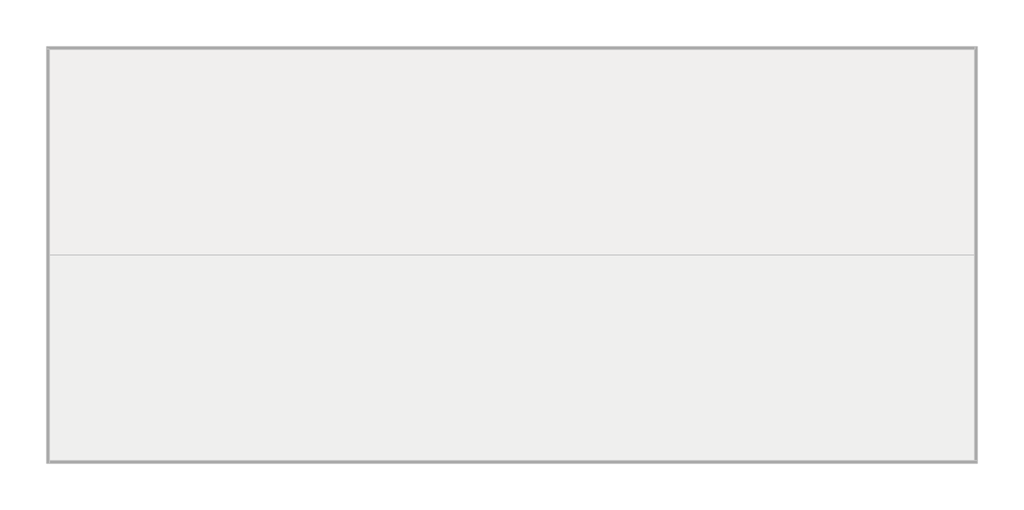
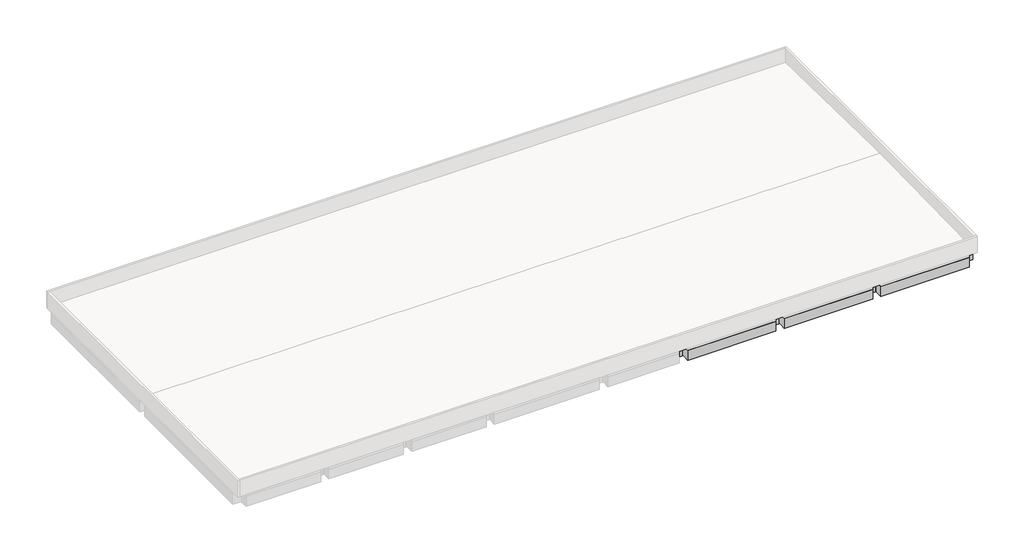
# One storey, part 2 of 2: 37 beams.
"""IFC4 building model written with IfcOpenShell, lengths in millimetres."""

from ifc_helpers import new_model, si_unit, origin, place, context, project, spatial, faceted_brep, element, save

model = new_model("IFC4")

# Units and contexts
model_context = context("Model", 3, world=origin())
ifc_project = project(units=[si_unit("LENGTHUNIT", "METRE", prefix="MILLI")], contexts=[model_context])

# Site, building, storey
site = spatial("IfcSite", under=ifc_project)
building = spatial("IfcBuilding", under=site)
storey = spatial("IfcBuildingStorey", under=building, Name="TOC", Elevation=7649.9618634)

# Beams
placement = place(None, origin())
element("IfcBeam", 1, ObjectType="RC Beam_Rectangular : H_SB_AR_S16_B600xH900_RG9", at=placement, inside=storey, context=model_context, shape_type="Brep", body=[
    faceted_brep([(300.0, 24199.5208589, 6749.9618634), (300.0, 23749.5208589, 6749.9618634), (300.0, 23599.5208589, 6749.9618634), (300.0, 23599.5208589, 7499.9618634), (300.0, 24199.5208589, 7499.9618634), (5700.0, 23599.5208589, 6749.9618634), (5700.0, 23749.5208589, 6749.9618634), (5700.0, 24199.5208589, 6749.9618634), (5700.0, 24199.5208589, 7499.9618634), (5700.0, 23599.5208589, 7499.9618634), (2800.0, 23599.5208589, 7499.9618634), (3200.0, 23599.5208589, 7499.9618634), (2800.0, 23599.5208589, 6749.9618634), (3200.0, 23599.5208589, 6749.9618634)], [[[0, 1, 2, 3, 4]], [[5, 6, 7, 8, 9]], [[4, 3, 10, 11, 9, 8]], [[2, 12, 13, 5, 9, 11, 10, 3]], [[2, 1, 0, 7, 6, 5, 13, 12]], [[7, 0, 4, 8]]]),
])
element("IfcBeam", 2, ObjectType="RC Beam_Rectangular : H_SB_AR_S16_B600xH900_RG9", at=placement, inside=storey, context=model_context, shape_type="Brep", body=[
    faceted_brep([(6300.0, 24199.5208589, 6749.9618634), (6300.0, 23749.5208589, 6749.9618634), (6300.0, 23599.5208589, 6749.9618634), (6300.0, 23599.5208589, 7499.9618634), (6300.0, 24199.5208589, 7499.9618634), (11700.0, 23599.5208589, 6749.9618634), (11700.0, 23749.5208589, 6749.9618634), (11700.0, 24199.5208589, 6749.9618634), (11700.0, 24199.5208589, 7499.9618634), (11700.0, 23599.5208589, 7499.9618634), (8800.0, 23599.5208589, 7499.9618634), (9200.0, 23599.5208589, 7499.9618634), (8800.0, 23599.5208589, 6749.9618634), (9200.0, 23599.5208589, 6749.9618634)], [[[0, 1, 2, 3, 4]], [[5, 6, 7, 8, 9]], [[4, 3, 10, 11, 9, 8]], [[2, 12, 13, 5, 9, 11, 10, 3]], [[2, 1, 0, 7, 6, 5, 13, 12]], [[7, 0, 4, 8]]]),
])
element("IfcBeam", 3, ObjectType="RC Beam_Rectangular : H_SB_AR_S16_B600xH900_RG9", at=placement, inside=storey, context=model_context, shape_type="Brep", body=[
    faceted_brep([(12300.0, 24199.5208589, 6749.9618634), (12300.0, 23749.5208589, 6749.9618634), (12300.0, 23599.5208589, 6749.9618634), (12300.0, 23599.5208589, 7499.9618634), (12300.0, 24199.5208589, 7499.9618634), (17700.0, 23599.5208589, 6749.9618634), (17700.0, 23749.5208589, 6749.9618634), (17700.0, 24199.5208589, 6749.9618634), (17700.0, 24199.5208589, 7499.9618634), (17700.0, 23599.5208589, 7499.9618634), (14800.0, 23599.5208589, 7499.9618634), (15200.0, 23599.5208589, 7499.9618634), (14800.0, 23599.5208589, 6749.9618634), (15200.0, 23599.5208589, 6749.9618634)], [[[0, 1, 2, 3, 4]], [[5, 6, 7, 8, 9]], [[4, 3, 10, 11, 9, 8]], [[2, 12, 13, 5, 9, 11, 10, 3]], [[2, 1, 0, 7, 6, 5, 13, 12]], [[7, 0, 4, 8]]]),
])
element("IfcBeam", 4, ObjectType="RC Beam_Rectangular : H_SB_AR_S16_B600xH900_RG9", at=placement, inside=storey, context=model_context, shape_type="Brep", body=[
    faceted_brep([(18300.0, 24199.5208589, 6749.9618634), (18300.0, 23749.5208589, 6749.9618634), (18300.0, 23599.5208589, 6749.9618634), (18300.0, 23599.5208589, 7499.9618634), (18300.0, 24199.5208589, 7499.9618634), (25900.0, 23599.5208589, 6749.9618634), (25900.0, 23749.5208589, 6749.9618634), (25900.0, 24199.5208589, 6749.9618634), (25900.0, 24199.5208589, 7499.9618634), (25900.0, 23599.5208589, 7499.9618634), (21800.0, 23599.5208589, 7499.9618634), (22400.0, 23599.5208589, 7499.9618634), (21800.0, 23599.5208589, 6749.9618634), (22400.0, 23599.5208589, 6749.9618634)], [[[0, 1, 2, 3, 4]], [[5, 6, 7, 8, 9]], [[4, 3, 10, 11, 9, 8]], [[2, 12, 13, 5, 9, 11, 10, 3]], [[2, 1, 0, 7, 6, 5, 13, 12]], [[7, 0, 4, 8]]]),
])
element("IfcBeam", 5, ObjectType="RC Beam_Rectangular : H_SB_AR_S16_B600xH900_RG9", at=placement, inside=storey, context=model_context, shape_type="Brep", body=[
    faceted_brep([(26500.0, 24199.5208589, 6749.9618634), (26500.0, 23749.5208589, 6749.9618634), (26500.0, 23599.5208589, 6749.9618634), (26500.0, 23599.5208589, 7499.9618634), (26500.0, 24199.5208589, 7499.9618634), (31700.0, 23599.5208589, 6749.9618634), (31700.0, 23749.5208589, 6749.9618634), (31700.0, 24199.5208589, 6749.9618634), (31700.0, 24199.5208589, 7499.9618634), (31700.0, 23599.5208589, 7499.9618634), (28800.0, 23599.5208589, 7499.9618634), (29400.0, 23599.5208589, 7499.9618634), (28800.0, 23599.5208589, 6749.9618634), (29400.0, 23599.5208589, 6749.9618634)], [[[0, 1, 2, 3, 4]], [[5, 6, 7, 8, 9]], [[4, 3, 10, 11, 9, 8]], [[2, 12, 13, 5, 9, 11, 10, 3]], [[2, 1, 0, 7, 6, 5, 13, 12]], [[7, 0, 4, 8]]]),
])
element("IfcBeam", 6, ObjectType="RC Beam_Rectangular : H_SB_AR_S16_B600xH900_RG9", at=placement, inside=storey, context=model_context, shape_type="Brep", body=[
    faceted_brep([(32300.0, 24199.5208589, 6749.9618634), (32300.0, 23749.5208589, 6749.9618634), (32300.0, 23599.5208589, 6749.9618634), (32300.0, 23599.5208589, 7499.9618634), (32300.0, 24199.5208589, 7499.9618634), (38700.0, 23599.5208589, 6749.9618634), (38700.0, 23749.5208589, 6749.9618634), (38700.0, 24199.5208589, 6749.9618634), (38700.0, 24199.5208589, 7499.9618634), (38700.0, 23599.5208589, 7499.9618634), (33250.0, 23599.5208589, 7499.9618634), (33450.0, 23599.5208589, 7499.9618634), (35200.0, 23599.5208589, 7499.9618634), (35800.0, 23599.5208589, 7499.9618634), (35200.0, 23599.5208589, 6749.9618634), (35800.0, 23599.5208589, 6749.9618634)], [[[0, 1, 2, 3, 4]], [[5, 6, 7, 8, 9]], [[4, 3, 10, 11, 12, 13, 9, 8]], [[2, 14, 15, 5, 9, 13, 12, 11, 10, 3]], [[2, 1, 0, 7, 6, 5, 15, 14]], [[7, 0, 4, 8]]]),
])
element("IfcBeam", 7, ObjectType="RC Beam_Rectangular : H_SB_AR_S16_B600xH900_RG9", at=placement, inside=storey, context=model_context, shape_type="Brep", body=[
    faceted_brep([(39300.0, 24199.5208589, 6749.9618634), (39300.0, 23749.5208589, 6749.9618634), (39300.0, 23599.5208589, 6749.9618634), (39300.0, 23599.5208589, 7499.9618634), (39300.0, 24199.5208589, 7499.9618634), (45700.0, 23599.5208589, 6749.9618634), (45700.0, 23749.5208589, 6749.9618634), (45700.0, 24199.5208589, 6749.9618634), (45700.0, 24199.5208589, 7499.9618634), (45700.0, 23599.5208589, 7499.9618634), (42200.0, 23599.5208589, 7499.9618634), (42800.0, 23599.5208589, 7499.9618634), (43500.0, 23599.5208589, 7499.9618634), (43700.0, 23599.5208589, 7499.9618634), (42200.0, 23599.5208589, 6749.9618634), (42800.0, 23599.5208589, 6749.9618634)], [[[0, 1, 2, 3, 4]], [[5, 6, 7, 8, 9]], [[4, 3, 10, 11, 12, 13, 9, 8]], [[2, 14, 15, 5, 9, 13, 12, 11, 10, 3]], [[2, 1, 0, 7, 6, 5, 15, 14]], [[7, 0, 4, 8]]]),
])
element("IfcBeam", 8, ObjectType="RC Beam_Rectangular : H_SB_AR_S16_B600xH900_RG9", at=placement, inside=storey, context=model_context, shape_type="Brep", body=[
    faceted_brep([(46300.0, 24199.5208589, 6749.9618634), (46300.0, 23749.5208589, 6749.9618634), (46300.0, 23599.5208589, 6749.9618634), (46300.0, 23599.5208589, 7499.9618634), (46300.0, 24199.5208589, 7499.9618634), (52700.0, 23599.5208589, 6749.9618634), (52700.0, 23749.5208589, 6749.9618634), (52700.0, 24199.5208589, 6749.9618634), (52700.0, 24199.5208589, 7499.9618634), (52700.0, 23599.5208589, 7499.9618634), (48900.0, 23599.5208589, 7499.9618634), (49100.0, 23599.5208589, 7499.9618634), (49200.0, 23599.5208589, 7499.9618634), (49800.0, 23599.5208589, 7499.9618634), (52574.0, 23599.5208589, 7499.9618634), (49200.0, 23599.5208589, 6749.9618634), (49800.0, 23599.5208589, 6749.9618634)], [[[0, 1, 2, 3, 4]], [[5, 6, 7, 8, 9]], [[4, 3, 10, 11, 12, 13, 14, 9, 8]], [[2, 15, 16, 5, 9, 14, 13, 12, 11, 10, 3]], [[2, 1, 0, 7, 6, 5, 16, 15]], [[7, 0, 4, 8]]]),
])
element("IfcBeam", 9, ObjectType="RC Beam_Rectangular : H_SB_AR_S16_B600xH900_RG5", at=placement, inside=storey, context=model_context, shape_type="Brep", body=[
    faceted_brep([(32300.0, 8599.5208589, 6749.9618634), (32300.0, 8399.5208589, 6749.9618634), (32300.0, 7999.5208589, 6749.9618634), (32300.0, 7999.5208589, 7499.9618634), (32300.0, 8599.5208589, 7499.9618634), (38700.0, 7999.5208589, 6749.9618634), (38700.0, 8599.5208589, 6749.9618634), (38700.0, 8599.5208589, 7499.9618634), (38700.0, 7999.5208589, 7499.9618634), (35200.0, 7999.5208589, 7499.9618634), (35800.0, 7999.5208589, 7499.9618634), (36500.0, 7999.5208589, 7499.9618634), (36700.0, 7999.5208589, 7499.9618634), (36700.0, 8599.5208589, 7499.9618634), (36500.0, 8599.5208589, 7499.9618634), (35800.0, 8599.5208589, 7499.9618634), (35200.0, 8599.5208589, 7499.9618634), (33450.0, 8599.5208589, 7499.9618634), (33250.0, 8599.5208589, 7499.9618634), (35200.0, 7999.5208589, 6749.9618634), (35800.0, 7999.5208589, 6749.9618634), (36500.0, 7999.5208589, 6749.9618634), (36700.0, 7999.5208589, 6749.9618634), (35200.0, 8599.5208589, 6749.9618634), (35800.0, 8599.5208589, 6749.9618634), (36500.0, 8599.5208589, 6749.9618634), (36700.0, 8599.5208589, 6749.9618634)], [[[0, 1, 2, 3, 4]], [[5, 6, 7, 8]], [[4, 3, 9, 10, 11, 12, 8, 7, 13, 14, 15, 16, 17, 18]], [[2, 19, 20, 21, 22, 5, 8, 12, 11, 10, 9, 3]], [[2, 1, 0, 23, 24, 25, 26, 6, 5, 22, 21, 20, 19]], [[6, 26, 25, 24, 23, 0, 4, 18, 17, 16, 15, 14, 13, 7]]]),
])
element("IfcBeam", 10, ObjectType="RC Beam_Rectangular : H_SB_AR_S16_B600xH900_RG5", at=placement, inside=storey, context=model_context, shape_type="Brep", body=[
    faceted_brep([(39300.0, 8599.5208589, 6749.9618634), (39300.0, 8404.5208589, 6749.9618634), (39300.0, 8204.5208589, 6749.9618634), (39300.0, 7999.5208589, 6749.9618634), (39300.0, 7999.5208589, 7499.9618634), (39300.0, 8599.5208589, 7499.9618634), (45700.0, 7999.5208589, 6749.9618634), (45700.0, 8399.5208589, 6749.9618634), (45700.0, 8599.5208589, 6749.9618634), (45700.0, 8599.5208589, 7499.9618634), (45700.0, 7999.5208589, 7499.9618634), (41925.0, 7999.5208589, 7499.9618634), (42125.0, 7999.5208589, 7499.9618634), (42200.0, 7999.5208589, 7499.9618634), (42800.0, 7999.5208589, 7499.9618634), (43200.0, 7999.5208589, 7499.9618634), (43400.0, 7999.5208589, 7499.9618634), (45440.0, 7999.5208589, 7499.9618634), (45640.0, 7999.5208589, 7499.9618634), (42800.0, 8599.5208589, 7499.9618634), (42200.0, 8599.5208589, 7499.9618634), (41925.0, 7999.5208589, 6749.9618634), (42125.0, 7999.5208589, 6749.9618634), (42200.0, 7999.5208589, 6749.9618634), (42800.0, 7999.5208589, 6749.9618634), (43200.0, 7999.5208589, 6749.9618634), (43400.0, 7999.5208589, 6749.9618634), (45440.0, 7999.5208589, 6749.9618634), (45640.0, 7999.5208589, 6749.9618634), (42200.0, 8599.5208589, 6749.9618634), (42800.0, 8599.5208589, 6749.9618634), (45440.0, 8599.5208589, 6749.9618634), (45640.0, 8599.5208589, 6749.9618634)], [[[0, 1, 2, 3, 4, 5]], [[6, 7, 8, 9, 10]], [[5, 4, 11, 12, 13, 14, 15, 16, 17, 18, 10, 9, 19, 20]], [[3, 21, 22, 23, 24, 25, 26, 27, 28, 6, 10, 18, 17, 16, 15, 14, 13, 12, 11, 4]], [[3, 2, 1, 0, 29, 30, 31, 32, 8, 7, 6, 28, 27, 26, 25, 24, 23, 22, 21]], [[8, 32, 31, 30, 29, 0, 5, 20, 19, 9]]]),
])
element("IfcBeam", 11, ObjectType="RC Beam_Rectangular : H_SB_AR_S16_B600xH900_RG5", at=placement, inside=storey, context=model_context, shape_type="Brep", body=[
    faceted_brep([(46300.0, 8599.5208589, 6749.9618634), (46300.0, 8399.5208589, 6749.9618634), (46300.0, 7999.5208589, 6749.9618634), (46300.0, 7999.5208589, 7499.9618634), (46300.0, 8599.5208589, 7499.9618634), (52700.0, 7999.5208589, 6749.9618634), (52700.0, 8399.5208589, 6749.9618634), (52700.0, 8599.5208589, 6749.9618634), (52700.0, 8599.5208589, 7499.9618634), (52700.0, 7999.5208589, 7499.9618634), (49200.0, 7999.5208589, 7499.9618634), (49800.0, 7999.5208589, 7499.9618634), (52574.0, 7999.5208589, 7499.9618634), (52574.0, 8599.5208589, 7499.9618634), (50725.0, 8599.5208589, 7499.9618634), (50525.0, 8599.5208589, 7499.9618634), (49800.0, 8599.5208589, 7499.9618634), (49200.0, 8599.5208589, 7499.9618634), (49200.0, 7999.5208589, 6749.9618634), (49800.0, 7999.5208589, 6749.9618634), (52574.0, 7999.5208589, 6749.9618634), (49200.0, 8599.5208589, 6749.9618634), (49800.0, 8599.5208589, 6749.9618634)], [[[0, 1, 2, 3, 4]], [[5, 6, 7, 8, 9]], [[4, 3, 10, 11, 12, 9, 8, 13, 14, 15, 16, 17]], [[2, 18, 19, 20, 5, 9, 12, 11, 10, 3]], [[2, 1, 0, 21, 22, 7, 6, 5, 20, 19, 18]], [[7, 22, 21, 0, 4, 17, 16, 15, 14, 13, 8]]]),
])
element("IfcBeam", 12, ObjectType="RC Beam_Rectangular : H_SB_AR_S16_B600xH900_RG9", at=placement, inside=storey, context=model_context, shape_type="Brep", body=[
    faceted_brep([(32300.0, 799.5208589, 6749.9618634), (32300.0, 649.5208589, 6749.9618634), (32300.0, 199.5208589, 6749.9618634), (32300.0, 199.5208589, 7499.9618634), (32300.0, 799.5208589, 7499.9618634), (38700.0, 199.5208589, 6749.9618634), (38700.0, 649.5208589, 6749.9618634), (38700.0, 799.5208589, 6749.9618634), (38700.0, 799.5208589, 7499.9618634), (38700.0, 199.5208589, 7499.9618634), (36700.0, 799.5208589, 7499.9618634), (36500.0, 799.5208589, 7499.9618634), (35800.0, 799.5208589, 7499.9618634), (35200.0, 799.5208589, 7499.9618634), (35200.0, 799.5208589, 6749.9618634), (35800.0, 799.5208589, 6749.9618634)], [[[0, 1, 2, 3, 4]], [[5, 6, 7, 8, 9]], [[4, 3, 9, 8, 10, 11, 12, 13]], [[2, 5, 9, 3]], [[2, 1, 0, 14, 15, 7, 6, 5]], [[7, 15, 14, 0, 4, 13, 12, 11, 10, 8]]]),
])
element("IfcBeam", 13, ObjectType="RC Beam_Rectangular : H_SB_AR_S16_B600xH900_RG9", at=placement, inside=storey, context=model_context, shape_type="Brep", body=[
    faceted_brep([(39300.0, 799.5208589, 6749.9618634), (39300.0, 649.5208589, 6749.9618634), (39300.0, 199.5208589, 6749.9618634), (39300.0, 199.5208589, 7499.9618634), (39300.0, 799.5208589, 7499.9618634), (45700.0, 199.5208589, 6749.9618634), (45700.0, 649.5208589, 6749.9618634), (45700.0, 799.5208589, 6749.9618634), (45700.0, 799.5208589, 7499.9618634), (45700.0, 199.5208589, 7499.9618634), (43400.0, 799.5208589, 7499.9618634), (43200.0, 799.5208589, 7499.9618634), (42800.0, 799.5208589, 7499.9618634), (42200.0, 799.5208589, 7499.9618634), (42200.0, 799.5208589, 6749.9618634), (42800.0, 799.5208589, 6749.9618634)], [[[0, 1, 2, 3, 4]], [[5, 6, 7, 8, 9]], [[4, 3, 9, 8, 10, 11, 12, 13]], [[2, 5, 9, 3]], [[2, 1, 0, 14, 15, 7, 6, 5]], [[7, 15, 14, 0, 4, 13, 12, 11, 10, 8]]]),
])
element("IfcBeam", 14, ObjectType="RC Beam_Rectangular : H_SB_AR_S16_B600xH900_RG9", at=placement, inside=storey, context=model_context, shape_type="Brep", body=[
    faceted_brep([(46300.0, 799.5208589, 6749.9618634), (46300.0, 649.5208589, 6749.9618634), (46300.0, 199.5208589, 6749.9618634), (46300.0, 199.5208589, 7499.9618634), (46300.0, 799.5208589, 7499.9618634), (52700.0, 199.5208589, 6749.9618634), (52700.0, 649.5208589, 6749.9618634), (52700.0, 799.5208589, 6749.9618634), (52700.0, 799.5208589, 7499.9618634), (52700.0, 199.5208589, 7499.9618634), (49800.0, 799.5208589, 7499.9618634), (49200.0, 799.5208589, 7499.9618634), (46800.0, 799.5208589, 7499.9618634), (46600.0, 799.5208589, 7499.9618634), (49200.0, 799.5208589, 6749.9618634), (49800.0, 799.5208589, 6749.9618634)], [[[0, 1, 2, 3, 4]], [[5, 6, 7, 8, 9]], [[4, 3, 9, 8, 10, 11, 12, 13]], [[2, 5, 9, 3]], [[2, 1, 0, 14, 15, 7, 6, 5]], [[7, 15, 14, 0, 4, 13, 12, 11, 10, 8]]]),
])
element("IfcBeam", 15, ObjectType="RC Beam_Rectangular : H_SB_AR_S16_B400xH900_RG1", at=placement, inside=storey, context=model_context, shape_type="Brep", body=[
    faceted_brep([(6200.0, 23599.5208589, 7499.9618634), (5800.0, 23599.5208589, 7499.9618634), (5800.0, 23473.5208589, 7499.9618634), (5800.0, 12499.5208589, 7499.9618634), (6200.0, 12499.5208589, 7499.9618634), (6200.0, 23473.5208589, 7499.9618634), (6200.0, 23599.5208589, 6749.9618634), (5800.0, 23599.5208589, 6749.9618634), (5800.0, 12499.5208589, 6749.9618634), (6200.0, 12499.5208589, 6749.9618634), (6200.0, 23473.5208589, 6749.9618634), (5800.0, 23473.5208589, 6749.9618634)], [[[0, 1, 2, 3, 4, 5]], [[6, 7, 1, 0]], [[8, 9, 4, 3]], [[9, 10, 6, 0, 5, 4]], [[8, 11, 7, 6, 10, 9]], [[7, 11, 8, 3, 2, 1]]]),
])
element("IfcBeam", 16, ObjectType="RC Beam_Rectangular : H_SB_AR_S16_B400xH900_RG1", at=placement, inside=storey, context=model_context, shape_type="Brep", body=[
    faceted_brep([(12200.0, 23599.5208589, 7499.9618634), (11800.0, 23599.5208589, 7499.9618634), (11800.0, 23473.5208589, 7499.9618634), (11800.0, 12499.5208589, 7499.9618634), (12200.0, 12499.5208589, 7499.9618634), (12200.0, 23473.5208589, 7499.9618634), (12200.0, 23599.5208589, 6749.9618634), (11800.0, 23599.5208589, 6749.9618634), (11800.0, 12499.5208589, 6749.9618634), (12200.0, 12499.5208589, 6749.9618634), (12200.0, 23473.5208589, 6749.9618634), (11800.0, 23473.5208589, 6749.9618634)], [[[0, 1, 2, 3, 4, 5]], [[6, 7, 1, 0]], [[8, 9, 4, 3]], [[9, 10, 6, 0, 5, 4]], [[9, 8, 11, 7, 6, 10]], [[7, 11, 8, 3, 2, 1]]]),
])
element("IfcBeam", 17, ObjectType="RC Beam_Rectangular : H_SB_AR_S16_B600xH900_RG1A", at=placement, inside=storey, context=model_context, shape_type="Brep", body=[
    faceted_brep([(17700.0, 12499.5208589, 6749.9618634), (18100.0, 12499.5208589, 6749.9618634), (18300.0, 12499.5208589, 6749.9618634), (18300.0, 12499.5208589, 7499.9618634), (17700.0, 12499.5208589, 7499.9618634), (18300.0, 23473.5208589, 7499.9618634), (18300.0, 23599.5208589, 7499.9618634), (17700.0, 23599.5208589, 7499.9618634), (17700.0, 23473.5208589, 7499.9618634), (18300.0, 23599.5208589, 6749.9618634), (18100.0, 23599.5208589, 6749.9618634), (17700.0, 23599.5208589, 6749.9618634), (17700.0, 23473.5208589, 6749.9618634)], [[[0, 1, 2, 3, 4]], [[4, 3, 5, 6, 7, 8]], [[9, 10, 11, 7, 6]], [[2, 9, 6, 5, 3]], [[0, 12, 11, 10, 9, 2, 1]], [[11, 12, 0, 4, 8, 7]]]),
])
element("IfcBeam", 18, ObjectType="RC Beam_Rectangular : H_SB_AR_S16_B500xH900_RG2", at=placement, inside=storey, context=model_context, shape_type="Brep", body=[
    faceted_brep([(26450.0, 23599.5208589, 7499.9618634), (25950.0, 23599.5208589, 7499.9618634), (25950.0, 23473.5208589, 7499.9618634), (25950.0, 8599.5208589, 7499.9618634), (26450.0, 8599.5208589, 7499.9618634), (26450.0, 23473.5208589, 7499.9618634), (26450.0, 23599.5208589, 6749.9618634), (25950.0, 23599.5208589, 6749.9618634), (25950.0, 8599.5208589, 6749.9618634), (26450.0, 8599.5208589, 6749.9618634), (26450.0, 23473.5208589, 6749.9618634), (25950.0, 23473.5208589, 6749.9618634)], [[[0, 1, 2, 3, 4, 5]], [[6, 7, 1, 0]], [[8, 9, 4, 3]], [[9, 10, 6, 0, 5, 4]], [[6, 10, 9, 8, 11, 7]], [[7, 11, 8, 3, 2, 1]]]),
])
element("IfcBeam", 19, ObjectType="RC Beam_Rectangular : H_SB_AR_S16_B500xH900_RG3", at=placement, inside=storey, context=model_context, shape_type="Brep", body=[
    faceted_brep([(31750.0, 799.5208589, 7499.9618634), (32250.0, 799.5208589, 7499.9618634), (32250.0, 925.5208589, 7499.9618634), (32250.0, 7999.5208589, 7499.9618634), (31750.0, 7999.5208589, 7499.9618634), (31750.0, 799.5208589, 6749.9618634), (31900.0, 799.5208589, 6749.9618634), (32250.0, 799.5208589, 6749.9618634), (32250.0, 7999.5208589, 6749.9618634), (31900.0, 7999.5208589, 6749.9618634), (31750.0, 7999.5208589, 6749.9618634), (32250.0, 925.5208589, 6749.9618634)], [[[0, 1, 2, 3, 4]], [[5, 6, 7, 1, 0]], [[8, 9, 10, 4, 3]], [[7, 11, 8, 3, 2, 1]], [[5, 10, 9, 8, 11, 7, 6]], [[10, 5, 0, 4]]]),
])
element("IfcBeam", 20, ObjectType="RC Beam_Rectangular : H_SB_AR_S16_B500xH900_RG2", at=placement, inside=storey, context=model_context, shape_type="Brep", body=[
    faceted_brep([(32250.0, 23599.5208589, 7499.9618634), (31750.0, 23599.5208589, 7499.9618634), (31750.0, 23473.5208589, 7499.9618634), (31750.0, 8599.5208589, 7499.9618634), (32250.0, 8599.5208589, 7499.9618634), (32250.0, 23473.5208589, 7499.9618634), (32250.0, 23599.5208589, 6749.9618634), (31750.0, 23599.5208589, 6749.9618634), (31750.0, 8599.5208589, 6749.9618634), (32250.0, 8599.5208589, 6749.9618634), (32250.0, 23473.5208589, 6749.9618634), (31750.0, 23473.5208589, 6749.9618634)], [[[0, 1, 2, 3, 4, 5]], [[6, 7, 1, 0]], [[8, 9, 4, 3]], [[9, 10, 6, 0, 5, 4]], [[8, 11, 7, 6, 10, 9]], [[7, 11, 8, 3, 2, 1]]]),
])
element("IfcBeam", 21, ObjectType="RC Beam_Rectangular : H_SB_AR_S16_B500xH900_RG3", at=placement, inside=storey, context=model_context, shape_type="Brep", body=[
    faceted_brep([(38750.0, 799.5208589, 7499.9618634), (39250.0, 799.5208589, 7499.9618634), (39250.0, 925.5208589, 7499.9618634), (39250.0, 4649.5208589, 7499.9618634), (39250.0, 4849.5208589, 7499.9618634), (39250.0, 7999.5208589, 7499.9618634), (38750.0, 7999.5208589, 7499.9618634), (38750.0, 3543.8249516, 7499.9618634), (38750.0, 3343.8249516, 7499.9618634), (38750.0, 925.5208589, 7499.9618634), (38750.0, 799.5208589, 6749.9618634), (38900.0, 799.5208589, 6749.9618634), (39100.0, 799.5208589, 6749.9618634), (39250.0, 799.5208589, 6749.9618634), (39250.0, 7999.5208589, 6749.9618634), (39100.0, 7999.5208589, 6749.9618634), (38900.0, 7999.5208589, 6749.9618634), (38750.0, 7999.5208589, 6749.9618634), (39250.0, 925.5208589, 6749.9618634), (39250.0, 4649.5208589, 6749.9618634), (39250.0, 4849.5208589, 6749.9618634), (38750.0, 925.5208589, 6749.9618634), (38750.0, 3343.8249516, 6749.9618634), (38750.0, 3543.8249516, 6749.9618634)], [[[0, 1, 2, 3, 4, 5, 6, 7, 8, 9]], [[10, 11, 12, 13, 1, 0]], [[14, 15, 16, 17, 6, 5]], [[13, 18, 19, 20, 14, 5, 4, 3, 2, 1]], [[10, 21, 22, 23, 17, 16, 15, 14, 20, 19, 18, 13, 12, 11]], [[17, 23, 22, 21, 10, 0, 9, 8, 7, 6]]]),
])
element("IfcBeam", 22, ObjectType="RC Beam_Rectangular : H_SB_AR_S16_B500xH900_RG2", at=placement, inside=storey, context=model_context, shape_type="Brep", body=[
    faceted_brep([(39250.0, 23599.5208589, 7499.9618634), (38750.0, 23599.5208589, 7499.9618634), (38750.0, 23473.5208589, 7499.9618634), (38750.0, 11149.5208589, 7499.9618634), (38750.0, 10949.5208589, 7499.9618634), (38750.0, 8599.5208589, 7499.9618634), (39250.0, 8599.5208589, 7499.9618634), (39250.0, 10949.5208589, 7499.9618634), (39250.0, 11149.5208589, 7499.9618634), (39250.0, 23473.5208589, 7499.9618634), (39250.0, 23599.5208589, 6749.9618634), (38750.0, 23599.5208589, 6749.9618634), (38750.0, 8599.5208589, 6749.9618634), (39250.0, 8599.5208589, 6749.9618634), (39250.0, 10949.5208589, 6749.9618634), (39250.0, 11149.5208589, 6749.9618634), (39250.0, 23473.5208589, 6749.9618634), (38750.0, 10949.5208589, 6749.9618634), (38750.0, 11149.5208589, 6749.9618634), (38750.0, 23473.5208589, 6749.9618634)], [[[0, 1, 2, 3, 4, 5, 6, 7, 8, 9]], [[10, 11, 1, 0]], [[12, 13, 6, 5]], [[13, 14, 15, 16, 10, 0, 9, 8, 7, 6]], [[12, 17, 18, 19, 11, 10, 16, 15, 14, 13]], [[11, 19, 18, 17, 12, 5, 4, 3, 2, 1]]]),
])
element("IfcBeam", 23, ObjectType="RC Beam_Rectangular : H_SB_AR_S16_B500xH900_RG3", at=placement, inside=storey, context=model_context, shape_type="Brep", body=[
    faceted_brep([(45750.0, 799.5208589, 7499.9618634), (46250.0, 799.5208589, 7499.9618634), (46250.0, 925.5208589, 7499.9618634), (46250.0, 4649.5208589, 7499.9618634), (46250.0, 4849.5208589, 7499.9618634), (46250.0, 6599.5208589, 7499.9618634), (46250.0, 6799.5208589, 7499.9618634), (46250.0, 7999.5208589, 7499.9618634), (45750.0, 7999.5208589, 7499.9618634), (45750.0, 6799.5208589, 7499.9618634), (45750.0, 6599.5208589, 7499.9618634), (45750.0, 4849.5208589, 7499.9618634), (45750.0, 4649.5208589, 7499.9618634), (45750.0, 925.5208589, 7499.9618634), (45750.0, 799.5208589, 6749.9618634), (46250.0, 799.5208589, 6749.9618634), (46250.0, 7999.5208589, 6749.9618634), (45750.0, 7999.5208589, 6749.9618634), (46250.0, 925.5208589, 6749.9618634), (46250.0, 4649.5208589, 6749.9618634), (46250.0, 4849.5208589, 6749.9618634), (46250.0, 6599.5208589, 6749.9618634), (46250.0, 6799.5208589, 6749.9618634), (45750.0, 925.5208589, 6749.9618634), (45750.0, 4649.5208589, 6749.9618634), (45750.0, 4849.5208589, 6749.9618634), (45750.0, 6599.5208589, 6749.9618634), (45750.0, 6799.5208589, 6749.9618634)], [[[0, 1, 2, 3, 4, 5, 6, 7, 8, 9, 10, 11, 12, 13]], [[14, 15, 1, 0]], [[16, 17, 8, 7]], [[15, 18, 19, 20, 21, 22, 16, 7, 6, 5, 4, 3, 2, 1]], [[14, 23, 24, 25, 26, 27, 17, 16, 22, 21, 20, 19, 18, 15]], [[17, 27, 26, 25, 24, 23, 14, 0, 13, 12, 11, 10, 9, 8]]]),
])
element("IfcBeam", 24, ObjectType="RC Beam_Rectangular : H_SB_AR_S16_B500xH900_RG2", at=placement, inside=storey, context=model_context, shape_type="Brep", body=[
    faceted_brep([(46250.0, 23599.5208589, 7499.9618634), (45750.0, 23599.5208589, 7499.9618634), (45750.0, 19999.5208589, 7499.9618634), (45750.0, 19799.5208589, 7499.9618634), (45750.0, 11149.5208589, 7499.9618634), (45750.0, 10949.5208589, 7499.9618634), (45750.0, 8599.5208589, 7499.9618634), (46250.0, 8599.5208589, 7499.9618634), (46250.0, 10149.5208589, 7499.9618634), (46250.0, 10349.5208589, 7499.9618634), (46250.0, 13899.5208589, 7499.9618634), (46250.0, 14099.5208589, 7499.9618634), (46250.0, 15214.5208589, 7499.9618634), (46250.0, 15414.5208589, 7499.9618634), (46250.0, 16549.5208589, 7499.9618634), (46250.0, 16749.5208589, 7499.9618634), (46250.0, 18399.5208589, 7499.9618634), (46250.0, 18599.5208589, 7499.9618634), (46250.0, 19799.5208589, 7499.9618634), (46250.0, 19999.5208589, 7499.9618634), (46250.0, 23473.5208589, 7499.9618634), (46250.0, 23599.5208589, 6749.9618634), (45900.0, 23599.5208589, 6749.9618634), (45750.0, 23599.5208589, 6749.9618634), (45750.0, 8599.5208589, 6749.9618634), (46250.0, 8599.5208589, 6749.9618634), (46250.0, 10149.5208589, 6749.9618634), (46250.0, 10349.5208589, 6749.9618634), (46250.0, 13899.5208589, 6749.9618634), (46250.0, 14099.5208589, 6749.9618634), (46250.0, 15214.5208589, 6749.9618634), (46250.0, 15414.5208589, 6749.9618634), (46250.0, 16549.5208589, 6749.9618634), (46250.0, 16749.5208589, 6749.9618634), (46250.0, 18399.5208589, 6749.9618634), (46250.0, 18599.5208589, 6749.9618634), (46250.0, 19799.5208589, 6749.9618634), (46250.0, 19999.5208589, 6749.9618634), (46250.0, 23473.5208589, 6749.9618634), (45750.0, 10949.5208589, 6749.9618634), (45750.0, 11149.5208589, 6749.9618634), (45750.0, 19799.5208589, 6749.9618634), (45750.0, 19999.5208589, 6749.9618634)], [[[0, 1, 2, 3, 4, 5, 6, 7, 8, 9, 10, 11, 12, 13, 14, 15, 16, 17, 18, 19, 20]], [[21, 22, 23, 1, 0]], [[24, 25, 7, 6]], [[25, 26, 27, 28, 29, 30, 31, 32, 33, 34, 35, 36, 37, 38, 21, 0, 20, 19, 18, 17, 16, 15, 14, 13, 12, 11, 10, 9, 8, 7]], [[24, 39, 40, 41, 42, 23, 22, 21, 38, 37, 36, 35, 34, 33, 32, 31, 30, 29, 28, 27, 26, 25]], [[23, 42, 41, 40, 39, 24, 6, 5, 4, 3, 2, 1]]]),
])
element("IfcBeam", 25, ObjectType="RC Beam_Rectangular : H_SB_AR_S16_B600xH900_RG8", at=placement, inside=storey, context=model_context, shape_type="Brep", body=[
    faceted_brep([(53300.0, 7999.5208589, 6749.9618634), (52850.0, 7999.5208589, 6749.9618634), (52700.0, 7999.5208589, 6749.9618634), (52700.0, 7999.5208589, 7499.9618634), (53300.0, 7999.5208589, 7499.9618634), (52700.0, 799.5208589, 6749.9618634), (52850.0, 799.5208589, 6749.9618634), (53300.0, 799.5208589, 6749.9618634), (53300.0, 799.5208589, 7499.9618634), (52700.0, 799.5208589, 7499.9618634), (52700.0, 925.5208589, 7499.9618634)], [[[0, 1, 2, 3, 4]], [[5, 6, 7, 8, 9]], [[4, 3, 10, 9, 8]], [[7, 0, 4, 8]], [[2, 1, 0, 7, 6, 5]], [[2, 5, 9, 10, 3]]]),
])
element("IfcBeam", 26, ObjectType="RC Beam_Rectangular : H_SB_AR_S16_B600xH900_RG7", at=placement, inside=storey, context=model_context, shape_type="Brep", body=[
    faceted_brep([(53300.0, 23599.5208589, 6749.9618634), (52850.0, 23599.5208589, 6749.9618634), (52700.0, 23599.5208589, 6749.9618634), (52700.0, 23599.5208589, 7499.9618634), (53300.0, 23599.5208589, 7499.9618634), (52700.0, 8599.5208589, 6749.9618634), (52850.0, 8599.5208589, 6749.9618634), (53300.0, 8599.5208589, 6749.9618634), (53300.0, 8599.5208589, 7499.9618634), (52700.0, 8599.5208589, 7499.9618634), (52700.0, 18599.5208589, 7499.9618634), (52700.0, 18399.5208589, 7499.9618634), (52700.0, 14099.5208589, 7499.9618634), (52700.0, 13899.5208589, 7499.9618634), (52700.0, 11774.5208589, 7499.9618634), (52700.0, 11574.5208589, 7499.9618634)], [[[0, 1, 2, 3, 4]], [[5, 6, 7, 8, 9]], [[4, 3, 10, 11, 12, 13, 14, 15, 9, 8]], [[7, 0, 4, 8]], [[2, 1, 0, 7, 6, 5]], [[2, 5, 9, 15, 14, 13, 12, 11, 10, 3]]]),
])
element("IfcBeam", 27, ObjectType="RC Beam_Rectangular : H_SB_AR_S16_B400xH900_RB1", at=placement, inside=storey, context=model_context, shape_type="Brep", body=[
    faceted_brep([(2800.0, 23599.5208589, 6749.9618634), (2800.0, 23473.5208589, 6749.9618634), (2800.0, 12499.5208589, 6749.9618634), (2800.0, 12499.5208589, 7499.9618634), (2800.0, 23473.5208589, 7499.9618634), (2800.0, 23599.5208589, 7499.9618634), (3200.0, 12499.5208589, 6749.9618634), (3200.0, 23599.5208589, 6749.9618634), (3200.0, 23473.5208589, 6749.9618634), (3200.0, 23599.5208589, 7499.9618634), (3200.0, 23473.5208589, 7499.9618634), (3200.0, 12499.5208589, 7499.9618634)], [[[0, 1, 2, 3, 4, 5]], [[6, 2, 1, 0, 7, 8]], [[6, 8, 7, 9, 10, 11]], [[2, 6, 11, 3]], [[7, 0, 5, 9]], [[5, 4, 3, 11, 10, 9]]]),
])
element("IfcBeam", 28, ObjectType="RC Beam_Rectangular : H_SB_AR_S16_B400xH900_RB1", at=placement, inside=storey, context=model_context, shape_type="Brep", body=[
    faceted_brep([(8800.0, 23599.5208589, 6749.9618634), (8800.0, 23473.5208589, 6749.9618634), (8800.0, 12499.5208589, 6749.9618634), (8800.0, 12499.5208589, 7499.9618634), (8800.0, 23473.5208589, 7499.9618634), (8800.0, 23599.5208589, 7499.9618634), (9200.0, 12499.5208589, 6749.9618634), (9200.0, 23599.5208589, 6749.9618634), (9200.0, 23473.5208589, 6749.9618634), (9200.0, 23599.5208589, 7499.9618634), (9200.0, 23473.5208589, 7499.9618634), (9200.0, 12499.5208589, 7499.9618634)], [[[0, 1, 2, 3, 4, 5]], [[6, 2, 1, 0, 7, 8]], [[6, 8, 7, 9, 10, 11]], [[2, 6, 11, 3]], [[7, 0, 5, 9]], [[5, 4, 3, 11, 10, 9]]]),
])
element("IfcBeam", 29, ObjectType="RC Beam_Rectangular : H_SB_AR_S16_B400xH900_RB1", at=placement, inside=storey, context=model_context, shape_type="Brep", body=[
    faceted_brep([(14800.0, 23599.5208589, 6749.9618634), (14800.0, 23473.5208589, 6749.9618634), (14800.0, 12499.5208589, 6749.9618634), (14800.0, 12499.5208589, 7499.9618634), (14800.0, 23473.5208589, 7499.9618634), (14800.0, 23599.5208589, 7499.9618634), (15200.0, 12499.5208589, 6749.9618634), (15200.0, 23599.5208589, 6749.9618634), (15200.0, 23473.5208589, 6749.9618634), (15200.0, 23599.5208589, 7499.9618634), (15200.0, 23473.5208589, 7499.9618634), (15200.0, 12499.5208589, 7499.9618634)], [[[0, 1, 2, 3, 4, 5]], [[6, 2, 1, 0, 7, 8]], [[6, 8, 7, 9, 10, 11]], [[2, 6, 11, 3]], [[7, 0, 5, 9]], [[5, 4, 3, 11, 10, 9]]]),
])
element("IfcBeam", 30, ObjectType="RC Beam_Rectangular : H_SB_AR_S16_B600xH900_RB2", at=placement, inside=storey, context=model_context, shape_type="Brep", body=[
    faceted_brep([(21800.0, 23599.5208589, 6749.9618634), (21800.0, 23473.5208589, 6749.9618634), (21800.0, 8599.5208589, 6749.9618634), (21800.0, 8599.5208589, 7499.9618634), (21800.0, 23473.5208589, 7499.9618634), (21800.0, 23599.5208589, 7499.9618634), (22400.0, 8599.5208589, 6749.9618634), (22400.0, 23599.5208589, 6749.9618634), (22400.0, 23473.5208589, 6749.9618634), (22400.0, 23599.5208589, 7499.9618634), (22400.0, 23473.5208589, 7499.9618634), (22400.0, 8599.5208589, 7499.9618634)], [[[0, 1, 2, 3, 4, 5]], [[6, 2, 1, 0, 7, 8]], [[6, 8, 7, 9, 10, 11]], [[2, 6, 11, 3]], [[7, 0, 5, 9]], [[5, 4, 3, 11, 10, 9]]]),
])
element("IfcBeam", 31, ObjectType="RC Beam_Rectangular : H_SB_AR_S16_B600xH900_RB2", at=placement, inside=storey, context=model_context, shape_type="Brep", body=[
    faceted_brep([(28800.0, 23599.5208589, 6749.9618634), (28800.0, 23473.5208589, 6749.9618634), (28800.0, 8599.5208589, 6749.9618634), (28800.0, 8599.5208589, 7499.9618634), (28800.0, 23473.5208589, 7499.9618634), (28800.0, 23599.5208589, 7499.9618634), (29400.0, 8599.5208589, 6749.9618634), (29400.0, 23599.5208589, 6749.9618634), (29400.0, 23473.5208589, 6749.9618634), (29400.0, 23599.5208589, 7499.9618634), (29400.0, 23473.5208589, 7499.9618634), (29400.0, 8599.5208589, 7499.9618634)], [[[0, 1, 2, 3, 4, 5]], [[6, 2, 1, 0, 7, 8]], [[6, 8, 7, 9, 10, 11]], [[2, 6, 11, 3]], [[7, 0, 5, 9]], [[5, 4, 3, 11, 10, 9]]]),
])
element("IfcBeam", 32, ObjectType="RC Beam_Rectangular : H_SB_AR_S16_B600xH900_RB2", at=placement, inside=storey, context=model_context, shape_type="Brep", body=[
    faceted_brep([(35200.0, 23599.5208589, 6749.9618634), (35200.0, 23473.5208589, 6749.9618634), (35200.0, 8599.5208589, 6749.9618634), (35200.0, 8599.5208589, 7499.9618634), (35200.0, 23473.5208589, 7499.9618634), (35200.0, 23599.5208589, 7499.9618634), (35800.0, 8599.5208589, 6749.9618634), (35800.0, 23599.5208589, 6749.9618634), (35800.0, 23473.5208589, 6749.9618634), (35800.0, 23599.5208589, 7499.9618634), (35800.0, 23473.5208589, 7499.9618634), (35800.0, 8599.5208589, 7499.9618634)], [[[0, 1, 2, 3, 4, 5]], [[6, 2, 1, 0, 7, 8]], [[6, 8, 7, 9, 10, 11]], [[2, 6, 11, 3]], [[7, 0, 5, 9]], [[5, 4, 3, 11, 10, 9]]]),
])
element("IfcBeam", 33, ObjectType="RC Beam_Rectangular : H_SB_AR_S16_B600xH900_RB3", at=placement, inside=storey, context=model_context, shape_type="Brep", body=[
    faceted_brep([(35200.0, 7999.5208589, 6749.9618634), (35200.0, 925.5208589, 6749.9618634), (35200.0, 799.5208589, 6749.9618634), (35200.0, 799.5208589, 7499.9618634), (35200.0, 925.5208589, 7499.9618634), (35200.0, 7999.5208589, 7499.9618634), (35800.0, 7999.5208589, 6749.9618634), (35800.0, 925.5208589, 6749.9618634), (35800.0, 799.5208589, 6749.9618634), (35800.0, 7999.5208589, 7499.9618634), (35800.0, 925.5208589, 7499.9618634), (35800.0, 799.5208589, 7499.9618634)], [[[0, 1, 2, 3, 4, 5]], [[0, 6, 7, 8, 2, 1]], [[8, 7, 6, 9, 10, 11]], [[6, 0, 5, 9]], [[2, 8, 11, 3]], [[5, 4, 3, 11, 10, 9]]]),
])
element("IfcBeam", 34, ObjectType="RC Beam_Rectangular : H_SB_AR_S16_B600xH900_RB2", at=placement, inside=storey, context=model_context, shape_type="Brep", body=[
    faceted_brep([(42200.0, 23599.5208589, 6749.9618634), (42200.0, 23473.5208589, 6749.9618634), (42200.0, 11149.5208589, 6749.9618634), (42200.0, 10949.5208589, 6749.9618634), (42200.0, 8599.5208589, 6749.9618634), (42200.0, 8599.5208589, 7499.9618634), (42200.0, 10949.5208589, 7499.9618634), (42200.0, 11149.5208589, 7499.9618634), (42200.0, 23473.5208589, 7499.9618634), (42200.0, 23599.5208589, 7499.9618634), (42800.0, 8599.5208589, 6749.9618634), (42800.0, 23599.5208589, 6749.9618634), (42800.0, 23473.5208589, 6749.9618634), (42800.0, 11149.5208589, 6749.9618634), (42800.0, 10949.5208589, 6749.9618634), (42800.0, 23599.5208589, 7499.9618634), (42800.0, 23473.5208589, 7499.9618634), (42800.0, 11149.5208589, 7499.9618634), (42800.0, 10949.5208589, 7499.9618634), (42800.0, 8599.5208589, 7499.9618634)], [[[0, 1, 2, 3, 4, 5, 6, 7, 8, 9]], [[10, 4, 3, 2, 1, 0, 11, 12, 13, 14]], [[10, 14, 13, 12, 11, 15, 16, 17, 18, 19]], [[4, 10, 19, 5]], [[11, 0, 9, 15]], [[9, 8, 7, 6, 5, 19, 18, 17, 16, 15]]]),
])
element("IfcBeam", 35, ObjectType="RC Beam_Rectangular : H_SB_AR_S16_B600xH900_RB3", at=placement, inside=storey, context=model_context, shape_type="Brep", body=[
    faceted_brep([(42200.0, 7999.5208589, 6749.9618634), (42200.0, 6274.5208589, 6749.9618634), (42200.0, 6074.5208589, 6749.9618634), (42200.0, 4849.5208589, 6749.9618634), (42200.0, 4649.5208589, 6749.9618634), (42200.0, 925.5208589, 6749.9618634), (42200.0, 799.5208589, 6749.9618634), (42200.0, 799.5208589, 7499.9618634), (42200.0, 925.5208589, 7499.9618634), (42200.0, 4649.5208589, 7499.9618634), (42200.0, 4849.5208589, 7499.9618634), (42200.0, 6074.5208589, 7499.9618634), (42200.0, 6274.5208589, 7499.9618634), (42200.0, 7999.5208589, 7499.9618634), (42800.0, 7999.5208589, 6749.9618634), (42800.0, 6274.5208589, 6749.9618634), (42800.0, 6074.5208589, 6749.9618634), (42800.0, 4849.5208589, 6749.9618634), (42800.0, 4649.5208589, 6749.9618634), (42800.0, 925.5208589, 6749.9618634), (42800.0, 799.5208589, 6749.9618634), (42800.0, 7999.5208589, 7499.9618634), (42800.0, 6274.5208589, 7499.9618634), (42800.0, 6074.5208589, 7499.9618634), (42800.0, 4849.5208589, 7499.9618634), (42800.0, 4649.5208589, 7499.9618634), (42800.0, 925.5208589, 7499.9618634), (42800.0, 799.5208589, 7499.9618634)], [[[0, 1, 2, 3, 4, 5, 6, 7, 8, 9, 10, 11, 12, 13]], [[0, 14, 15, 16, 17, 18, 19, 20, 6, 5, 4, 3, 2, 1]], [[20, 19, 18, 17, 16, 15, 14, 21, 22, 23, 24, 25, 26, 27]], [[14, 0, 13, 21]], [[6, 20, 27, 7]], [[13, 12, 11, 10, 9, 8, 7, 27, 26, 25, 24, 23, 22, 21]]]),
])
element("IfcBeam", 36, ObjectType="RC Beam_Rectangular : H_SB_AR_S16_B600xH900_RB2", at=placement, inside=storey, context=model_context, shape_type="Brep", body=[
    faceted_brep([(49200.0, 23599.5208589, 6749.9618634), (49200.0, 23473.5208589, 6749.9618634), (49200.0, 18599.5208589, 6749.9618634), (49200.0, 18399.5208589, 6749.9618634), (49200.0, 14099.5208589, 6749.9618634), (49200.0, 13899.5208589, 6749.9618634), (49200.0, 10349.5208589, 6749.9618634), (49200.0, 10149.5208589, 6749.9618634), (49200.0, 8599.5208589, 6749.9618634), (49200.0, 8599.5208589, 7499.9618634), (49200.0, 10149.5208589, 7499.9618634), (49200.0, 10349.5208589, 7499.9618634), (49200.0, 13899.5208589, 7499.9618634), (49200.0, 14099.5208589, 7499.9618634), (49200.0, 18399.5208589, 7499.9618634), (49200.0, 18599.5208589, 7499.9618634), (49200.0, 23473.5208589, 7499.9618634), (49200.0, 23599.5208589, 7499.9618634), (49800.0, 8599.5208589, 6749.9618634), (49800.0, 23599.5208589, 6749.9618634), (49800.0, 23473.5208589, 6749.9618634), (49800.0, 18599.5208589, 6749.9618634), (49800.0, 18399.5208589, 6749.9618634), (49800.0, 14099.5208589, 6749.9618634), (49800.0, 13899.5208589, 6749.9618634), (49800.0, 10349.5208589, 6749.9618634), (49800.0, 10149.5208589, 6749.9618634), (49800.0, 23599.5208589, 7499.9618634), (49800.0, 23473.5208589, 7499.9618634), (49800.0, 18599.5208589, 7499.9618634), (49800.0, 18399.5208589, 7499.9618634), (49800.0, 14099.5208589, 7499.9618634), (49800.0, 13899.5208589, 7499.9618634), (49800.0, 10349.5208589, 7499.9618634), (49800.0, 10149.5208589, 7499.9618634), (49800.0, 8599.5208589, 7499.9618634)], [[[0, 1, 2, 3, 4, 5, 6, 7, 8, 9, 10, 11, 12, 13, 14, 15, 16, 17]], [[18, 8, 7, 6, 5, 4, 3, 2, 1, 0, 19, 20, 21, 22, 23, 24, 25, 26]], [[18, 26, 25, 24, 23, 22, 21, 20, 19, 27, 28, 29, 30, 31, 32, 33, 34, 35]], [[8, 18, 35, 9]], [[19, 0, 17, 27]], [[17, 16, 15, 14, 13, 12, 11, 10, 9, 35, 34, 33, 32, 31, 30, 29, 28, 27]]]),
])
element("IfcBeam", 37, ObjectType="RC Beam_Rectangular : H_SB_AR_S16_B600xH900_RB3", at=placement, inside=storey, context=model_context, shape_type="Brep", body=[
    faceted_brep([(49200.0, 7999.5208589, 6749.9618634), (49200.0, 925.5208589, 6749.9618634), (49200.0, 799.5208589, 6749.9618634), (49200.0, 799.5208589, 7499.9618634), (49200.0, 925.5208589, 7499.9618634), (49200.0, 7999.5208589, 7499.9618634), (49800.0, 7999.5208589, 6749.9618634), (49800.0, 925.5208589, 6749.9618634), (49800.0, 799.5208589, 6749.9618634), (49800.0, 7999.5208589, 7499.9618634), (49800.0, 925.5208589, 7499.9618634), (49800.0, 799.5208589, 7499.9618634)], [[[0, 1, 2, 3, 4, 5]], [[0, 6, 7, 8, 2, 1]], [[8, 7, 6, 9, 10, 11]], [[6, 0, 5, 9]], [[2, 8, 11, 3]], [[5, 4, 3, 11, 10, 9]]]),
])

save(model, "model.ifc")

# Revit data of these elements
# Type "RC Beam_Rectangular : H_SB_AR_S16_B600xH900_RG9"
#   중앙부 하부근 = ""
#   중앙부 상부근 = ""
#   중앙부 보조근 = ""
#   중앙부 늑근 = ""
#   외단부 하부근 = ""
#   외단부 상부근 = ""
#   외단부 보조근 = ""
#   외단부 늑근 = ""
#   부호 = "TG3"
#   내단부 하부근 = ""
#   내단부 상부근 = ""
#   내단부 보조근 = ""
#   내단부 늑근 = ""
#   ALL 하부근 = "3-D20"
#   ALL 상부근 = "3-D20"
#   ALL 보조근 = ""
#   ALL 늑근 = "2-D10 @120"
#   Width = 600 mm
#   Height = 900 mm
#   Length [instance default] = 1524 mm
#   b = 600 mm
#   h = 900 mm
#   hec_material3 [instance default] = none
#   hec_material2 [instance default] = none
#   hec_material1 [instance default] = none
#   Structural Material [instance default] = none
#   Assembly Code = ""
# Type "RC Beam_Rectangular : H_SB_AR_S16_B600xH900_RG5"
#   중앙부 하부근 = ""
#   중앙부 상부근 = ""
#   중앙부 보조근 = ""
#   중앙부 늑근 = ""
#   외단부 하부근 = ""
#   외단부 상부근 = ""
#   외단부 보조근 = ""
#   외단부 늑근 = ""
#   부호 = "TG3"
#   내단부 하부근 = ""
#   내단부 상부근 = ""
#   내단부 보조근 = ""
#   내단부 늑근 = ""
#   ALL 하부근 = "3-D20"
#   ALL 상부근 = "3-D20"
#   ALL 보조근 = ""
#   ALL 늑근 = "2-D10 @120"
#   Width = 600 mm
#   Height = 900 mm
#   Length [instance default] = 1524 mm
#   b = 600 mm
#   h = 900 mm
#   hec_material3 [instance default] = none
#   hec_material2 [instance default] = none
#   hec_material1 [instance default] = none
#   Structural Material [instance default] = none
#   Assembly Code = ""
# Type "RC Beam_Rectangular : H_SB_AR_S16_B400xH900_RG1"
#   중앙부 하부근 = ""
#   중앙부 상부근 = ""
#   중앙부 보조근 = ""
#   중앙부 늑근 = ""
#   외단부 하부근 = ""
#   외단부 상부근 = ""
#   외단부 보조근 = ""
#   외단부 늑근 = ""
#   부호 = "TG3"
#   내단부 하부근 = ""
#   내단부 상부근 = ""
#   내단부 보조근 = ""
#   내단부 늑근 = ""
#   ALL 하부근 = "3-D20"
#   ALL 상부근 = "3-D20"
#   ALL 보조근 = ""
#   ALL 늑근 = "2-D10 @120"
#   Width = 400 mm
#   Height = 900 mm
#   Length [instance default] = 1524 mm
#   b = 400 mm
#   h = 900 mm
#   hec_material3 [instance default] = none
#   hec_material2 [instance default] = none
#   hec_material1 [instance default] = none
#   Structural Material [instance default] = none
#   Assembly Code = ""
# Type "RC Beam_Rectangular : H_SB_AR_S16_B600xH900_RG1A"
#   중앙부 하부근 = ""
#   중앙부 상부근 = ""
#   중앙부 보조근 = ""
#   중앙부 늑근 = ""
#   외단부 하부근 = ""
#   외단부 상부근 = ""
#   외단부 보조근 = ""
#   외단부 늑근 = ""
#   부호 = "TG3"
#   내단부 하부근 = ""
#   내단부 상부근 = ""
#   내단부 보조근 = ""
#   내단부 늑근 = ""
#   ALL 하부근 = "3-D20"
#   ALL 상부근 = "3-D20"
#   ALL 보조근 = ""
#   ALL 늑근 = "2-D10 @120"
#   Width = 600 mm
#   Height = 900 mm
#   Length [instance default] = 1524 mm
#   b = 600 mm
#   h = 900 mm
#   hec_material3 [instance default] = none
#   hec_material2 [instance default] = none
#   hec_material1 [instance default] = none
#   Structural Material [instance default] = none
#   Assembly Code = ""
# Type "RC Beam_Rectangular : H_SB_AR_S16_B500xH900_RG2"
#   중앙부 하부근 = ""
#   중앙부 상부근 = ""
#   중앙부 보조근 = ""
#   중앙부 늑근 = ""
#   외단부 하부근 = ""
#   외단부 상부근 = ""
#   외단부 보조근 = ""
#   외단부 늑근 = ""
#   부호 = "TG3"
#   내단부 하부근 = ""
#   내단부 상부근 = ""
#   내단부 보조근 = ""
#   내단부 늑근 = ""
#   ALL 하부근 = "3-D20"
#   ALL 상부근 = "3-D20"
#   ALL 보조근 = ""
#   ALL 늑근 = "2-D10 @120"
#   Width = 500 mm
#   Height = 900 mm
#   Length [instance default] = 1524 mm
#   b = 500 mm
#   h = 900 mm
#   hec_material3 [instance default] = none
#   hec_material2 [instance default] = none
#   hec_material1 [instance default] = none
#   Structural Material [instance default] = none
#   Assembly Code = ""
# Type "RC Beam_Rectangular : H_SB_AR_S16_B500xH900_RG3"
#   중앙부 하부근 = ""
#   중앙부 상부근 = ""
#   중앙부 보조근 = ""
#   중앙부 늑근 = ""
#   외단부 하부근 = ""
#   외단부 상부근 = ""
#   외단부 보조근 = ""
#   외단부 늑근 = ""
#   부호 = "TG3"
#   내단부 하부근 = ""
#   내단부 상부근 = ""
#   내단부 보조근 = ""
#   내단부 늑근 = ""
#   ALL 하부근 = "3-D20"
#   ALL 상부근 = "3-D20"
#   ALL 보조근 = ""
#   ALL 늑근 = "2-D10 @120"
#   Width = 500 mm
#   Height = 900 mm
#   Length [instance default] = 1524 mm
#   b = 500 mm
#   h = 900 mm
#   hec_material3 [instance default] = none
#   hec_material2 [instance default] = none
#   hec_material1 [instance default] = none
#   Structural Material [instance default] = none
#   Assembly Code = ""
# Type "RC Beam_Rectangular : H_SB_AR_S16_B600xH900_RG8"
#   중앙부 하부근 = ""
#   중앙부 상부근 = ""
#   중앙부 보조근 = ""
#   중앙부 늑근 = ""
#   외단부 하부근 = ""
#   외단부 상부근 = ""
#   외단부 보조근 = ""
#   외단부 늑근 = ""
#   부호 = "TG3"
#   내단부 하부근 = ""
#   내단부 상부근 = ""
#   내단부 보조근 = ""
#   내단부 늑근 = ""
#   ALL 하부근 = "3-D20"
#   ALL 상부근 = "3-D20"
#   ALL 보조근 = ""
#   ALL 늑근 = "2-D10 @120"
#   Width = 600 mm
#   Height = 900 mm
#   Length [instance default] = 1524 mm
#   b = 600 mm
#   h = 900 mm
#   hec_material3 [instance default] = none
#   hec_material2 [instance default] = none
#   hec_material1 [instance default] = none
#   Structural Material [instance default] = none
#   Assembly Code = ""
# Type "RC Beam_Rectangular : H_SB_AR_S16_B600xH900_RG7"
#   중앙부 하부근 = ""
#   중앙부 상부근 = ""
#   중앙부 보조근 = ""
#   중앙부 늑근 = ""
#   외단부 하부근 = ""
#   외단부 상부근 = ""
#   외단부 보조근 = ""
#   외단부 늑근 = ""
#   부호 = "TG3"
#   내단부 하부근 = ""
#   내단부 상부근 = ""
#   내단부 보조근 = ""
#   내단부 늑근 = ""
#   ALL 하부근 = "3-D20"
#   ALL 상부근 = "3-D20"
#   ALL 보조근 = ""
#   ALL 늑근 = "2-D10 @120"
#   Width = 600 mm
#   Height = 900 mm
#   Length [instance default] = 1524 mm
#   b = 600 mm
#   h = 900 mm
#   hec_material3 [instance default] = none
#   hec_material2 [instance default] = none
#   hec_material1 [instance default] = none
#   Structural Material [instance default] = none
#   Assembly Code = ""
# Type "RC Beam_Rectangular : H_SB_AR_S16_B400xH900_RB1"
#   중앙부 하부근 = ""
#   중앙부 상부근 = ""
#   중앙부 보조근 = ""
#   중앙부 늑근 = ""
#   외단부 하부근 = ""
#   외단부 상부근 = ""
#   외단부 보조근 = ""
#   외단부 늑근 = ""
#   부호 = "TG3"
#   내단부 하부근 = ""
#   내단부 상부근 = ""
#   내단부 보조근 = ""
#   내단부 늑근 = ""
#   ALL 하부근 = "3-D20"
#   ALL 상부근 = "3-D20"
#   ALL 보조근 = ""
#   ALL 늑근 = "2-D10 @120"
#   Width = 400 mm
#   Height = 900 mm
#   Length [instance default] = 1524 mm
#   b = 400 mm
#   h = 900 mm
#   hec_material3 [instance default] = none
#   hec_material2 [instance default] = none
#   hec_material1 [instance default] = none
#   Structural Material [instance default] = none
#   Assembly Code = ""
# Type "RC Beam_Rectangular : H_SB_AR_S16_B600xH900_RB2"
#   중앙부 하부근 = ""
#   중앙부 상부근 = ""
#   중앙부 보조근 = ""
#   중앙부 늑근 = ""
#   외단부 하부근 = ""
#   외단부 상부근 = ""
#   외단부 보조근 = ""
#   외단부 늑근 = ""
#   부호 = "TG3"
#   내단부 하부근 = ""
#   내단부 상부근 = ""
#   내단부 보조근 = ""
#   내단부 늑근 = ""
#   ALL 하부근 = "3-D20"
#   ALL 상부근 = "3-D20"
#   ALL 보조근 = ""
#   ALL 늑근 = "2-D10 @120"
#   Width = 600 mm
#   Height = 900 mm
#   Length [instance default] = 1524 mm
#   b = 600 mm
#   h = 900 mm
#   hec_material3 [instance default] = none
#   hec_material2 [instance default] = none
#   hec_material1 [instance default] = none
#   Structural Material [instance default] = none
#   Assembly Code = ""
# Type "RC Beam_Rectangular : H_SB_AR_S16_B600xH900_RB3"
#   중앙부 하부근 = ""
#   중앙부 상부근 = ""
#   중앙부 보조근 = ""
#   중앙부 늑근 = ""
#   외단부 하부근 = ""
#   외단부 상부근 = ""
#   외단부 보조근 = ""
#   외단부 늑근 = ""
#   부호 = "TG3"
#   내단부 하부근 = ""
#   내단부 상부근 = ""
#   내단부 보조근 = ""
#   내단부 늑근 = ""
#   ALL 하부근 = "3-D20"
#   ALL 상부근 = "3-D20"
#   ALL 보조근 = ""
#   ALL 늑근 = "2-D10 @120"
#   Width = 600 mm
#   Height = 900 mm
#   Length [instance default] = 1524 mm
#   b = 600 mm
#   h = 900 mm
#   hec_material3 [instance default] = none
#   hec_material2 [instance default] = none
#   hec_material1 [instance default] = none
#   Structural Material [instance default] = none
#   Assembly Code = ""
# Elements 1, 2, 3, 4, 5, 6, 7, 8, 12, 13, 14 (IfcBeam, "RC Beam_Rectangular : H_SB_AR_S16_B600xH900_RG9")
#   Comments = ""
#   hec_material3 = none
#   hec_material2 = none
#   hec_material1 = none
#   Structural Material = Concrete - Cast-in-Place Concrete - 35 MPa
#   Phase Created = New Construction
#   Materials on its faces: "Concrete - Cast-in-Place Concrete - 35 MPa"
# Elements 9, 10, 11 (IfcBeam, "RC Beam_Rectangular : H_SB_AR_S16_B600xH900_RG5")
#   Comments = ""
#   hec_material3 = none
#   hec_material2 = none
#   hec_material1 = none
#   Structural Material = Concrete - Cast-in-Place Concrete - 35 MPa
#   Phase Created = New Construction
#   Materials on its faces: "Concrete - Cast-in-Place Concrete - 35 MPa"
# Elements 15, 16 (IfcBeam, "RC Beam_Rectangular : H_SB_AR_S16_B400xH900_RG1")
#   Comments = ""
#   hec_material3 = none
#   hec_material2 = none
#   hec_material1 = none
#   Structural Material = Concrete - Cast-in-Place Concrete - 35 MPa
#   Phase Created = New Construction
#   Materials on its faces: "Concrete - Cast-in-Place Concrete - 35 MPa"
# Element 17 (IfcBeam, "RC Beam_Rectangular : H_SB_AR_S16_B600xH900_RG1A")
#   Comments = ""
#   hec_material3 = none
#   hec_material2 = none
#   hec_material1 = none
#   Structural Material = Concrete - Cast-in-Place Concrete - 35 MPa
#   Phase Created = New Construction
#   Materials on its faces: "Concrete - Cast-in-Place Concrete - 35 MPa"
# Elements 18, 20, 22, 24 (IfcBeam, "RC Beam_Rectangular : H_SB_AR_S16_B500xH900_RG2")
#   Comments = ""
#   hec_material3 = none
#   hec_material2 = none
#   hec_material1 = none
#   Structural Material = Concrete - Cast-in-Place Concrete - 35 MPa
#   Phase Created = New Construction
#   Materials on its faces: "Concrete - Cast-in-Place Concrete - 35 MPa"
# Elements 19, 21, 23 (IfcBeam, "RC Beam_Rectangular : H_SB_AR_S16_B500xH900_RG3")
#   Comments = ""
#   hec_material3 = none
#   hec_material2 = none
#   hec_material1 = none
#   Structural Material = Concrete - Cast-in-Place Concrete - 35 MPa
#   Phase Created = New Construction
#   Materials on its faces: "Concrete - Cast-in-Place Concrete - 35 MPa"
# Element 25 (IfcBeam, "RC Beam_Rectangular : H_SB_AR_S16_B600xH900_RG8")
#   Comments = ""
#   hec_material3 = none
#   hec_material2 = none
#   hec_material1 = none
#   Structural Material = Concrete - Cast-in-Place Concrete - 35 MPa
#   Phase Created = New Construction
#   Materials on its faces: "Concrete - Cast-in-Place Concrete - 35 MPa"
# Element 26 (IfcBeam, "RC Beam_Rectangular : H_SB_AR_S16_B600xH900_RG7")
#   Comments = ""
#   hec_material3 = none
#   hec_material2 = none
#   hec_material1 = none
#   Structural Material = Concrete - Cast-in-Place Concrete - 35 MPa
#   Phase Created = New Construction
#   Materials on its faces: "Concrete - Cast-in-Place Concrete - 35 MPa"
# Elements 27, 28, 29 (IfcBeam, "RC Beam_Rectangular : H_SB_AR_S16_B400xH900_RB1")
#   hec_material3 = none
#   hec_material2 = none
#   hec_material1 = none
#   Structural Material = Concrete - Cast-in-Place Concrete - 35 MPa
#   Phase Created = New Construction
#   Materials on its faces: "Concrete - Cast-in-Place Concrete - 35 MPa"
# Elements 30, 31, 32, 34, 36 (IfcBeam, "RC Beam_Rectangular : H_SB_AR_S16_B600xH900_RB2")
#   hec_material3 = none
#   hec_material2 = none
#   hec_material1 = none
#   Structural Material = Concrete - Cast-in-Place Concrete - 35 MPa
#   Phase Created = New Construction
#   Materials on its faces: "Concrete - Cast-in-Place Concrete - 35 MPa"
# Elements 33, 35, 37 (IfcBeam, "RC Beam_Rectangular : H_SB_AR_S16_B600xH900_RB3")
#   hec_material3 = none
#   hec_material2 = none
#   hec_material1 = none
#   Structural Material = Concrete - Cast-in-Place Concrete - 35 MPa
#   Phase Created = New Construction
#   Materials on its faces: "Concrete - Cast-in-Place Concrete - 35 MPa"
# Materials
#   "Concrete - Cast-in-Place Concrete - 35 MPa": class "Concrete", colour RGB 192 192 192, transparency 0, Cost = 0
